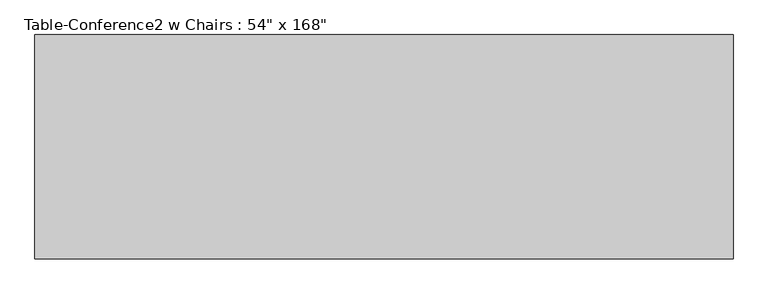
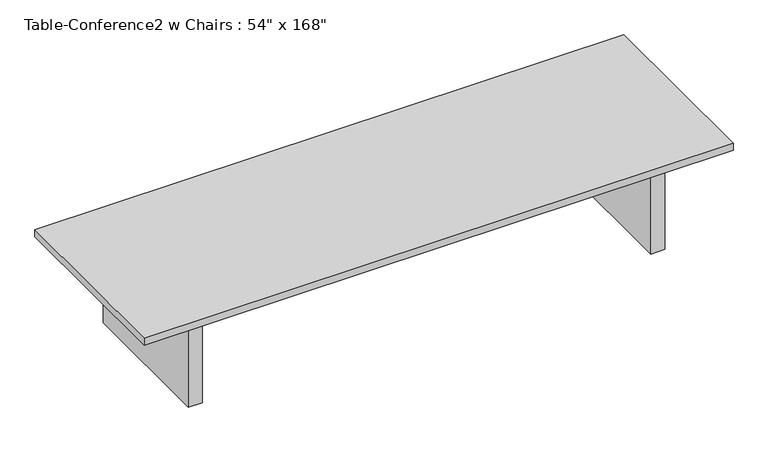
"""IFC4 building model written with IfcOpenShell, lengths in millimetres: furniture geometry."""

from ifc_helpers import new_model, si_unit, frame, origin, origin_with_axes, place, context, project, spatial, polyline, outline, extrude, source, transform, mapped, element, save


def furniture_afb95ac4(model_context):
    return source(origin(), model_context, "Body", "SweptSolid", [
        extrude(outline(polyline([(1625.6, 533.4), (1625.6, 495.3), (-1625.6, 495.3), (-1625.6, 533.4), (1625.6, 533.4)])), frame((0.0, 0.0, 609.6), z_axis=(0.0, 0.0, 1.0), x_axis=(1.0, 0.0, 0.0)), (0.0, 0.0, 1.0), 101.6),
        extrude(outline(polyline([(1625.6, -533.4), (-1625.6, -533.4), (-1625.6, -495.3), (1625.6, -495.3), (1625.6, -533.4)])), frame((0.0, 0.0, 609.6), z_axis=(0.0, 0.0, 1.0), x_axis=(1.0, 0.0, 0.0)), (0.0, 0.0, 1.0), 101.6),
        extrude(outline(polyline([(-1625.6, -533.4), (-1727.2, -533.4), (-1727.2, 533.4), (-1625.6, 533.4), (-1625.6, -533.4)])), origin_with_axes(), (0.0, 0.0, 1.0), 711.2),
        extrude(outline(polyline([(1727.2, -533.4), (1625.6, -533.4), (1625.6, 533.4), (1727.2, 533.4), (1727.2, -533.4)])), origin_with_axes(), (0.0, 0.0, 1.0), 711.2),
        extrude(outline(polyline([(2133.6, -685.8), (-2133.6, -685.8), (-2133.6, 685.8), (2133.6, 685.8), (2133.6, -685.8)])), frame((0.0, 0.0, 711.2), z_axis=(0.0, 0.0, 1.0), x_axis=(1.0, 0.0, 0.0)), (0.0, 0.0, 1.0), 50.8),
    ])


if __name__ == "__main__":
    model = new_model("IFC4")
    model_context = context("Model", 3, world=origin())
    ifc_project = project(units=[si_unit("LENGTHUNIT", "METRE", prefix="MILLI")], contexts=[model_context])
    site = spatial("IfcSite", under=ifc_project)
    building = spatial("IfcBuilding", under=site)
    placement = place(None, origin())
    furniture_shape = furniture_afb95ac4(model_context)
    element("IfcFurniture", 1, ObjectType="Table-Conference2 w Chairs : 54\" x 168\"", at=placement, inside=building, context=model_context, shape_type="MappedRepresentation", body=[
        mapped(furniture_shape, transform((0.0, 0.0, 0.0), x_axis=(1.0, 0.0, 0.0), y_axis=(0.0, 1.0, 0.0), z_axis=(0.0, 0.0, 1.0))),
    ])
    save(model, "model.ifc")

# Revit data of these elements
# Type "Table-Conference2 w Chairs : 54\" x 168\""
#   Type IfcGUID = "2u0XNFrAPALBFZCv81fqia"
#   Assembly Code = "E2020200"
#   Description = "Seating 14-16"
#   Height = 0.762 m
#   Length = 4.2672 m
#   Width = 1.3716 m
#   Number Of Chairs One Side = 6
#   Number Of Chairs = 14
#   Material = Wood - Cherry
#   Default Elevation = 0
# Element 1 (IfcFurniture, "Table-Conference2 w Chairs : 54\" x 168\"")
#   Materials on its faces: "Wood - Cherry"
# Materials
#   "Wood - Cherry": class "Wood", colour RGB 226 177 128, transparency 0
